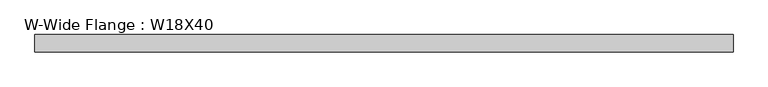
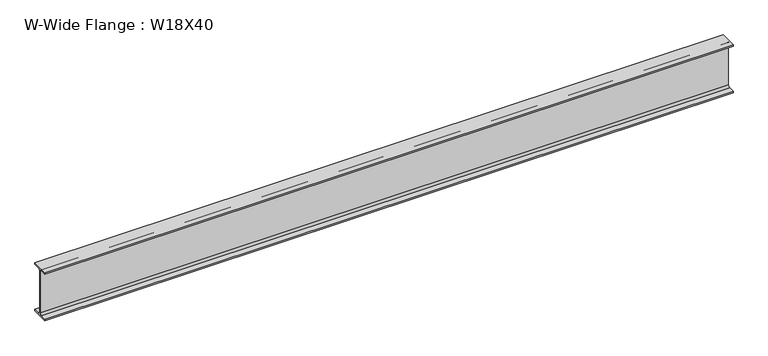
"""IFC4 building model written with IfcOpenShell, lengths in millimetres: beam geometry, W-Wide Flange : W18X40."""

from ifc_helpers import new_model, si_unit, point, frame, frame_2d, origin, place, context, project, spatial, polyline, circle_curve, trimmed, segment, composite_curve, outline, extrude, source, transform, mapped, element, save


def w_wide_flange_w18x40_1bcbd53f(model_context):
    return source(origin(), model_context, "Body", "SweptSolid", [
        extrude(outline(composite_curve([segment(polyline([(76.454, -213.995), (76.454, -227.33), (-76.454, -227.33), (-76.454, -213.995), (-20.828, -213.995)]), True, "CONTINUOUS"), segment(trimmed(circle_curve(frame_2d((-20.828, -197.1675)), 16.8275), [point((-20.828, -213.995))], [point((-4.0005, -197.1675))], True, "CARTESIAN"), True, "CONTINUOUS"), segment(polyline([(-4.0005, -197.1675), (-4.0005, 197.1675)]), True, "CONTINUOUS"), segment(trimmed(circle_curve(frame_2d((-20.828, 197.1675)), 16.8275), [point((-4.0005, 197.1675))], [point((-20.828, 213.995))], True, "CARTESIAN"), True, "CONTINUOUS"), segment(polyline([(-20.828, 213.995), (-76.454, 213.995), (-76.454, 227.33), (76.454, 227.33), (76.454, 213.995), (20.828, 213.995)]), True, "CONTINUOUS"), segment(trimmed(circle_curve(frame_2d((20.828, 197.1675)), 16.8275), [point((20.828, 213.995))], [point((4.0005, 197.1675))], True, "CARTESIAN"), True, "CONTINUOUS"), segment(polyline([(4.0005, 197.1675), (4.0005, -197.1675)]), True, "CONTINUOUS"), segment(trimmed(circle_curve(frame_2d((20.828, -197.1675)), 16.8275), [point((4.0005, -197.1675))], [point((20.828, -213.995))], True, "CARTESIAN"), True, "CONTINUOUS"), segment(polyline([(20.828, -213.995), (76.454, -213.995)]), True, "CONTINUOUS")], self_intersect=False)), frame((-3084.83, 0.0, 0.0), z_axis=(1.0, 0.0, 0.0), x_axis=(0.0, 1.0, 0.0)), (0.0, 0.0, 1.0), 6169.66),
    ])


if __name__ == "__main__":
    model = new_model("IFC4")
    model_context = context("Model", 3, world=origin())
    ifc_project = project(units=[si_unit("LENGTHUNIT", "METRE", prefix="MILLI")], contexts=[model_context])
    site = spatial("IfcSite", under=ifc_project)
    building = spatial("IfcBuilding", under=site)
    placement = place(None, origin())
    w_wide_flange_w18x40_shape = w_wide_flange_w18x40_1bcbd53f(model_context)
    element("IfcBeam", 1, ObjectType="W-Wide Flange : W18X40", at=placement, inside=building, context=model_context, shape_type="MappedRepresentation", body=[
        mapped(w_wide_flange_w18x40_shape, transform((0.0, 0.0, 0.0), x_axis=(1.0, 0.0, 0.0), y_axis=(0.0, 1.0, 0.0), z_axis=(0.0, 0.0, 1.0))),
    ])
    save(model, "model.ifc")

# Revit data of these elements
# Type "W-Wide Flange : W18X40"
#   Assembly Code = "B10"
#   W = 40
#   Length [instance default] = 5' - 0"
#   bf = 0' - 6.02"
#   d = 1' - 5.9"
#   k = 0' - 1 3/16"
#   k2 = 0' - 0.6625"
#   tf = 0' - 0.525"
#   tw = 0' - 0.315"
#   A = 0.0819444 SF
#   Structural Material [instance default] = Steel ASTM A992
# Element 1 (IfcBeam, "W-Wide Flange : W18X40")
#   Materials on its faces: "Steel ASTM A992"
# Materials
#   "Steel ASTM A992": class "Metal", colour RGB 199 199 199, transparency 0, Description = "Structural steel 50ksi", Cost = 0
